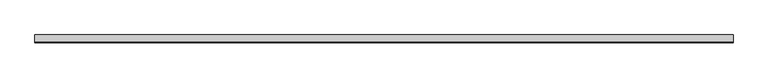
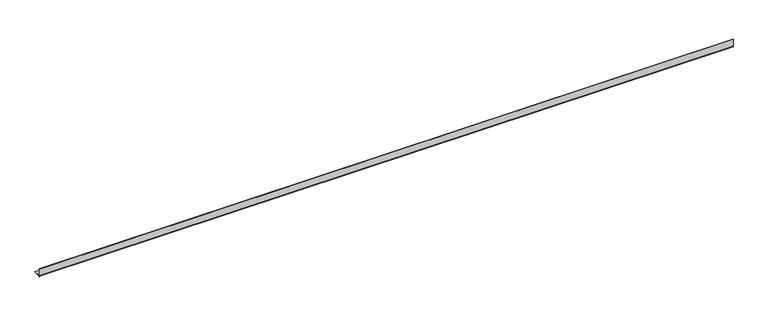
"""IFC4 building model written with IfcOpenShell, lengths in millimetres: proxy geometry, Metal profile006 2190 : Metal profile006 2190."""

from ifc_helpers import new_model, si_unit, point, frame, frame_2d, origin, place, context, project, spatial, polyline, circle_curve, trimmed, segment, composite_curve, outline, extrude, source, transform, mapped, element, save


def generic_models_1d1ee282(model_context):
    return source(origin(), model_context, "Body", "SweptSolid", [
        extrude(outline(composite_curve([segment(polyline([(9577.6300834, 39534.2760589), (9577.6300834, 39513.122875), (9598.7832673, 39513.122875), (9598.7832673, 39511.842875), (9577.8803576, 39511.842875)]), True, "CONTINUOUS"), segment(trimmed(circle_curve(frame_2d((9576.9900834, 39512.482875)), 1.0964434), [point((9577.8803576, 39511.842875))], [point((9576.3500834, 39513.3731492))], False, "CARTESIAN"), True, "CONTINUOUS"), segment(polyline([(9576.3500834, 39513.3731492), (9576.3500834, 39534.2760589), (9577.6300834, 39534.2760589)]), True, "CONTINUOUS")], self_intersect=False)), frame((3694.2883192, 0.0, 0.0), z_axis=(1.0, 0.0, 0.0), x_axis=(0.0, 1.0, 0.0)), (0.0, 0.0, 1.0), 2000.0),
    ])


if __name__ == "__main__":
    model = new_model("IFC4")
    model_context = context("Model", 3, world=origin())
    ifc_project = project(units=[si_unit("LENGTHUNIT", "METRE", prefix="MILLI")], contexts=[model_context])
    site = spatial("IfcSite", under=ifc_project)
    building = spatial("IfcBuilding", under=site)
    placement = place(None, origin())
    generic_models_shape = generic_models_1d1ee282(model_context)
    element("IfcBuildingElementProxy", 1, Name="Metal profile006 2190 : Metal profile006 2190", ObjectType="Metal profile006 2190 : Metal profile006 2190", at=placement, inside=building, context=model_context, shape_type="MappedRepresentation", body=[
        mapped(generic_models_shape, transform((0.0, 0.0, 0.0), x_axis=(1.0, 0.0, 0.0), y_axis=(0.0, 1.0, 0.0), z_axis=(0.0, 0.0, 1.0))),
    ])
    save(model, "model.ifc")

# Revit data of these elements
# Type "Metal profile006 2190 : Metal profile006 2190"
#   NameOverride = "Metal profile006"
# Element 1 (IfcBuildingElementProxy, "Metal profile006 2190 : Metal profile006 2190")
#   Materials on its faces: "CORNER BEAD"
# Materials
#   "CORNER BEAD": class "Unassigned", colour RGB 255 241 0, transparency 0
